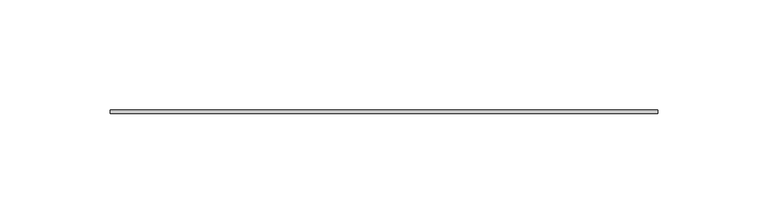
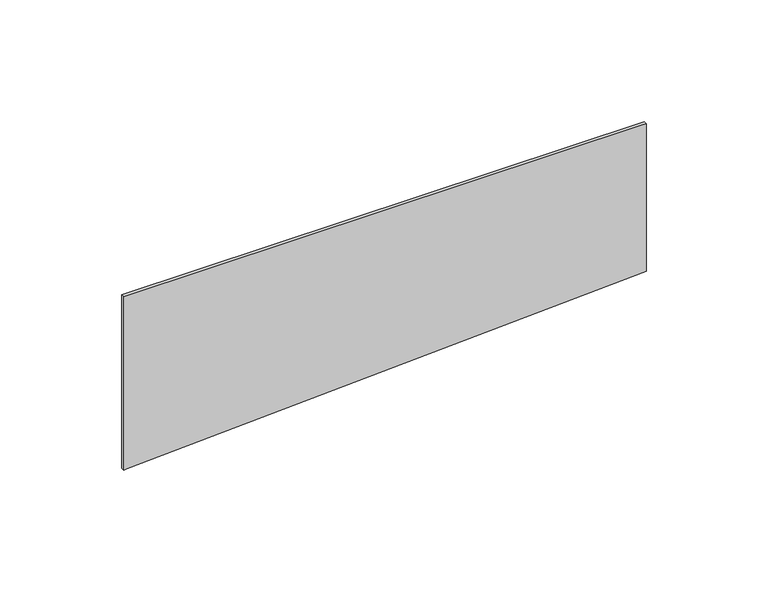
"""IFC4 building model written with IfcOpenShell, lengths in millimetres: proxy geometry, Generic Models 7:Generic Models 1:5:Generic Models 1:5 : Generic Models 7:Generic Models 1:337419:27 : Generic Models 7:Generic Models 1:5:Generic Models 1:5 : Generic Models 7:Generic Models 1:337419:311462."""

from ifc_helpers import new_model, si_unit, origin, place, context, project, spatial, faceted_brep, source, transform, mapped, element, save


def generic_models_11c69457(model_context):
    return source(origin(), model_context, "Body", "Brep", [
        faceted_brep([(667548.8992239, -568186.6413841, 6180.8221905), (667548.8992239, -568186.6413841, 6254.75), (667547.3117239, -568186.6413841, 6254.75), (667301.2492239, -568186.6413841, 6254.75), (667301.2492239, -568186.6413841, 6169.4330826), (667301.2492239, -568186.6413841, 6167.843404), (667302.8367239, -568186.6413841, 6167.9266014), (667548.8992239, -568185.1456181, 6180.8221905), (667301.2492239, -568185.1456181, 6167.843404), (667301.2492239, -568185.1456181, 6254.75), (667548.8992239, -568185.1456181, 6254.75)], [[[0, 1, 2, 3, 4, 5, 6]], [[7, 8, 9, 10]], [[0, 6, 5, 8, 7]], [[5, 4, 3, 9, 8]], [[1, 0, 7, 10]], [[3, 2, 1, 10, 9]]]),
    ])


if __name__ == "__main__":
    model = new_model("IFC4")
    model_context = context("Model", 3, world=origin())
    ifc_project = project(units=[si_unit("LENGTHUNIT", "METRE", prefix="MILLI")], contexts=[model_context])
    site = spatial("IfcSite", under=ifc_project)
    building = spatial("IfcBuilding", under=site)
    placement = place(None, origin())
    generic_models_shape = generic_models_11c69457(model_context)
    element("IfcBuildingElementProxy", 1, Name="Generic Models 7:Generic Models 1:5:Generic Models 1:5 : Generic Models 7:Generic Models 1:337419:27 : Generic Models 7:Generic Models 1:5:Generic Models 1:5 : Generic Models 7:Generic Models 1:337419:311462", ObjectType="Generic Models 7:Generic Models 1:5:Generic Models 1:5 : Generic Models 7:Generic Models 1:337419:27 : Generic Models 7:Generic Models 1:5:Generic Models 1:5 : Generic Models 7:Generic Models 1:337419:311462", at=placement, inside=building, context=model_context, shape_type="MappedRepresentation", body=[
        mapped(generic_models_shape, transform((0.0, 0.0, 0.0), x_axis=(1.0, 0.0, 0.0), y_axis=(0.0, 1.0, 0.0), z_axis=(0.0, 0.0, 1.0))),
    ])
    save(model, "model.ifc")

# Revit data of these elements
# Type "Generic Models 7:Generic Models 1:5:Generic Models 1:5 : Generic Models 7:Generic Models 1:337419:27 : Generic Models 7:Generic Models 1:5:Generic Models 1:5 : Generic Models 7:Generic Models 1:337419:311462"
#   NameOverride = "Generic Models 7:Generic Models 1:5:Generic Models 1:5 : Generic Models 7:Generic Models 1:337419:311462"
#   ObjectTypeOverride = "Generic Models 1:5 : Generic Models 7:Generic Models 1:337419"
#   Reference = "Generic Models 1"
#   Tag = "311462"
# Element 1 (IfcBuildingElementProxy, "Generic Models 7:Generic Models 1:5:Generic Models 1:5 : Generic Models 7:Generic Models 1:337419:27 : Generic Models 7:Generic Models 1:5:Generic Models 1:5 : Generic Models 7:Generic Models 1:337419:311462")
#   Materials on its faces: "SLOPED SHEET METAL COPING - (COLOR TO MATCH RESIN PANEL)"
# Materials
#   "SLOPED SHEET METAL COPING - (COLOR TO MATCH RESIN PANEL)": class "Generic", colour RGB 240 240 240, transparency 0, Keynote = "M07711300.01", Cost = 0
